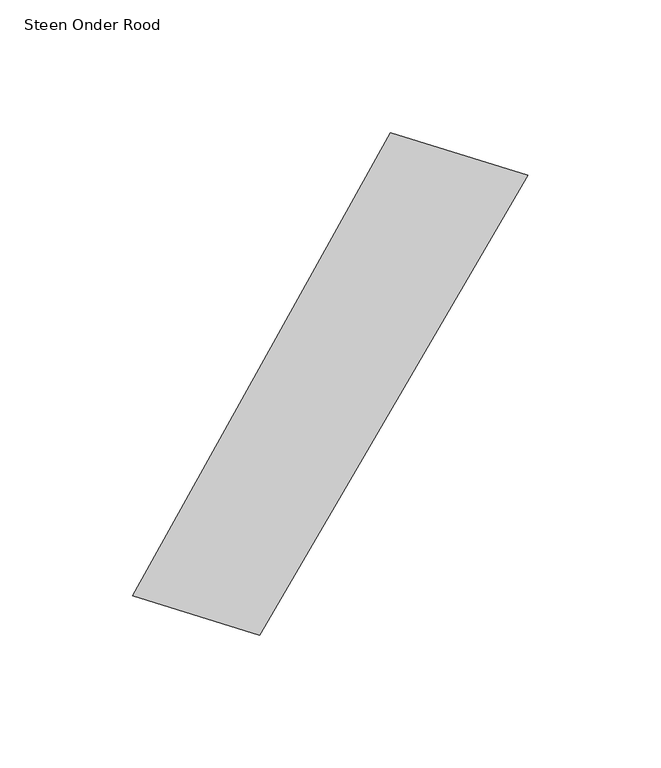
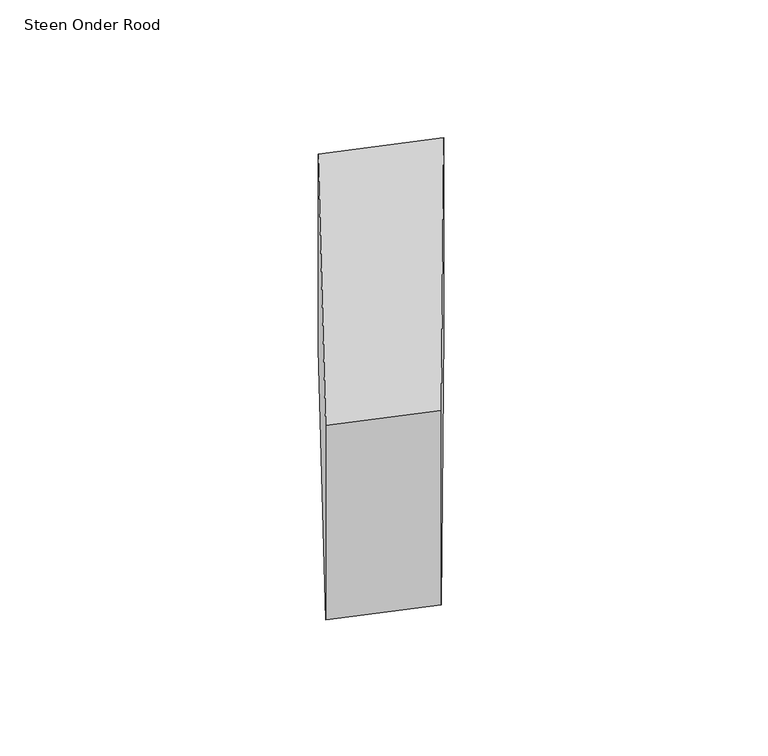
"""IFC4 building model written with IfcOpenShell, lengths in millimetres: proxy geometry, 00_GMA_steen_versie_4 : Steen Onder Rood."""

from ifc_helpers import new_model, si_unit, origin, origin_with_axes, place, context, project, spatial, polyline, outline, extrude, source, transform, mapped, element, save


def steen_onder_rood_2d7e6991(model_context):
    return source(origin(), model_context, "Body", "SweptSolid", [
        extrude(outline(polyline([(150.0751239, 154.4045945), (48.9532047, -18.5772423), (1.1829976, -3.8121714), (98.151695, 170.433064), (150.0751239, 154.4045945)])), origin_with_axes(), (0.0, 0.0, 1.0), 100.0),
    ])


if __name__ == "__main__":
    model = new_model("IFC4")
    model_context = context("Model", 3, world=origin())
    ifc_project = project(units=[si_unit("LENGTHUNIT", "METRE", prefix="MILLI")], contexts=[model_context])
    site = spatial("IfcSite", under=ifc_project)
    building = spatial("IfcBuilding", under=site)
    placement = place(None, origin())
    steen_onder_rood_shape = steen_onder_rood_2d7e6991(model_context)
    element("IfcBuildingElementProxy", 1, Name="00_GMA_steen_versie_4 : Steen Onder Rood", ObjectType="00_GMA_steen_versie_4 : Steen Onder Rood", at=placement, inside=building, context=model_context, shape_type="MappedRepresentation", body=[
        mapped(steen_onder_rood_shape, transform((0.0, 0.0, 0.0), x_axis=(1.0, 0.0, 0.0), y_axis=(0.0, 1.0, 0.0), z_axis=(0.0, 0.0, 1.0))),
    ])
    save(model, "model.ifc")

# Revit data of these elements
# Type "00_GMA_steen_versie_4 : Steen Onder Rood"
#   StootVoegHalfBoven [instance default] = 5 mm
#   StootVoegHalf [instance default] = 5 mm
#   StootVoegBreedteOnder = 10 mm
#   StootVoegBreedteBoven = 10 mm
#   Steendikte = 100 mm
#   LintVoegOnderHalf = 0 mm
#   LintVoegOnder = 0 mm
#   LintVoegBovenHalf = 5 mm
#   LintVoegBoven = 10 mm
#   materiaal = 21_steen_rood
#   MateriaalVoeg = none
#   Default Elevation = 0
# Element 1 (IfcBuildingElementProxy, "00_GMA_steen_versie_4 : Steen Onder Rood")
#   Materials on its faces: "21_steen_rood"
# Materials
#   "21_steen_rood": class "Unassigned", colour RGB 213 111 43, transparency 0, Cost = 0
